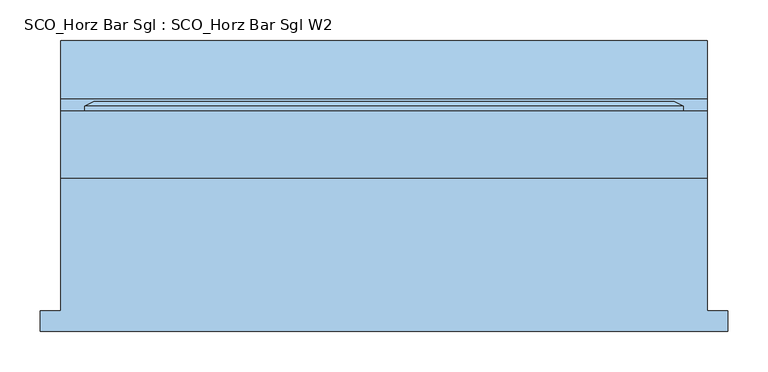
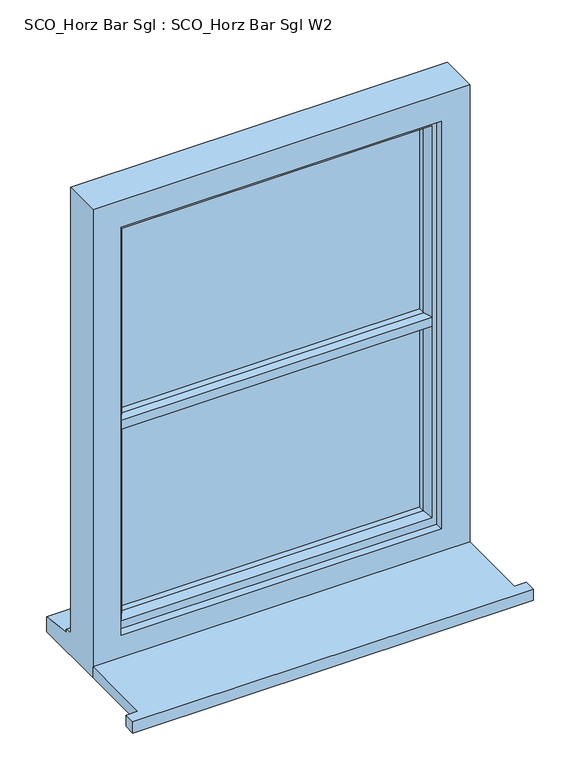
"""IFC4 building model written with IfcOpenShell, lengths in millimetres: window geometry, SCO_Horz Bar Sgl : SCO_Horz Bar Sgl W2."""

from ifc_helpers import new_model, si_unit, frame, origin, place, context, project, spatial, polyline, outline, extrude, faceted_brep, source, transform, mapped, element, save


def sco_horz_bar_sgl_sco_horz_bar_sgl_w2_7f5f4811(model_context):
    return source(origin(), model_context, "Body", "SolidModel", [
        extrude(outline(polyline([(-425.0, -191.5434322), (-425.0, -166.5434322), (-400.0, -166.5434322), (-400.0, -2.0434322), (400.0, -2.0434322), (400.0, -166.5434322), (425.0, -166.5434322), (425.0, -191.5434322), (-425.0, -191.5434322)])), frame((0.0, 0.0, 1060.0), z_axis=(0.0, 0.0, 1.0), x_axis=(1.0, 0.0, 0.0)), (0.0, 0.0, 1.0), 25.0),
        faceted_brep([(-400.0, -2.0434322, 1060.0), (400.0, -2.0434322, 1060.0), (400.0, -2.0434322, 2110.0), (-400.0, -2.0434322, 2110.0), (-340.0, -2.0434322, 2050.0), (340.0, -2.0434322, 2050.0), (340.0, -2.0434322, 1135.0), (-340.0, -2.0434322, 1135.0), (-400.0, 80.9565678, 2110.0), (-400.0, 80.9565678, 1111.0), (-400.0, 95.9565678, 1109.68767), (-400.0, 95.9565678, 1104.7449676), (-400.0, 168.4565678, 1093.8088847), (-400.0, 168.4565678, 1060.0), (400.0, 80.9565678, 2110.0), (400.0, 80.9565678, 1111.0), (-360.0, 80.9565678, 2070.0), (-360.0, 80.9565678, 1123.0), (360.0, 80.9565678, 1123.0), (360.0, 80.9565678, 2070.0), (-360.0, 15.9565678, 2070.0), (-360.0, 15.9565678, 1123.0), (360.0, 15.9565678, 2070.0), (360.0, 15.9565678, 1123.0), (-340.0, 15.9565678, 2050.0), (-340.0, 15.9565678, 1135.0), (340.0, 15.9565678, 1135.0), (340.0, 15.9565678, 2050.0), (400.0, 168.4565678, 1060.0), (400.0, 168.4565678, 1093.8088847), (400.0, 95.9565678, 1104.7449676), (400.0, 95.9565678, 1109.68767)], [[[0, 1, 2, 3], [4, 5, 6, 7]], [[0, 3, 8, 9, 10, 11, 12, 13]], [[9, 8, 14, 15], [16, 17, 18, 19]], [[17, 16, 20, 21]], [[20, 22, 23, 21], [24, 25, 26, 27]], [[24, 4, 7, 25]], [[3, 2, 14, 8]], [[16, 19, 22, 20]], [[5, 4, 24, 27]], [[15, 14, 2, 1, 28, 29, 30, 31]], [[19, 18, 23, 22]], [[5, 27, 26, 6]], [[28, 1, 0, 13]], [[29, 28, 13, 12]], [[30, 29, 12, 11]], [[31, 30, 11, 10]], [[15, 31, 10, 9]], [[21, 23, 18, 17]], [[7, 6, 26, 25]]]),
        extrude(outline(polyline([(330.1480377, 44.9565678), (-330.0, 44.9565678), (-330.0, 68.9565678), (330.1480377, 68.9565678), (330.1480377, 44.9565678)])), frame((0.0, 0.0, 1153.0), z_axis=(0.0, 0.0, 1.0), x_axis=(1.0, 0.0, 0.0)), (0.0, 0.0, 1.0), 434.3307627),
        extrude(outline(polyline([(330.1480377, 44.9565678), (-330.0, 44.9565678), (-330.0, 68.9565678), (330.1480377, 68.9565678), (330.1480377, 44.9565678)])), frame((0.0, 0.0, 1597.6692373), z_axis=(0.0, 0.0, 1.0), x_axis=(1.0, 0.0, 0.0)), (0.0, 0.0, 1.0), 442.3307627),
        extrude(outline(polyline([(92.5035732, 1597.6692373), (92.5035732, 1587.3307627), (86.8277797, 1577.5), (68.9565678, 1577.5), (68.9565678, 1584.5), (44.9565678, 1584.5), (44.9565678, 1577.5), (30.4494677, 1577.5), (15.9565678, 1582.6480377), (15.9565678, 1602.3519623), (30.4494677, 1607.5), (44.9565678, 1607.5), (44.9565678, 1600.5), (68.9565678, 1600.5), (68.9565678, 1607.5), (86.8277797, 1607.5), (92.5035732, 1597.6692373)])), frame((-330.1480377, 0.0, 0.0), z_axis=(1.0, 0.0, 0.0), x_axis=(0.0, 1.0, 0.0)), (0.0, 0.0, 1.0), 660.2960754),
        faceted_brep([(-370.0, 80.9565678, 2072.0), (-370.0, 86.7300705, 2072.0), (-370.0, 86.7300705, 1113.0), (-370.0, 80.9565678, 1113.0), (-360.0, 15.9565678, 2062.0), (-360.0, 80.9565678, 2062.0), (-360.0, 80.9565678, 1123.0), (-360.0, 15.9565678, 1123.0), (-320.0, 30.4494677, 2022.0), (-330.1480377, 15.9565678, 2032.1480377), (-330.1480377, 15.9565678, 1152.8519623), (-320.0, 30.4494677, 1163.0), (-320.0, 44.9565678, 2022.0), (-320.0, 44.9565678, 1163.0), (-330.0, 68.9565678, 2032.0), (-330.0, 44.9565678, 2032.0), (-330.0, 44.9565678, 1153.0), (-330.0, 68.9565678, 1153.0), (-320.0, 86.7300705, 2022.0), (-320.0, 68.9565678, 2022.0), (-320.0, 68.9565678, 1163.0), (-320.0, 86.7300705, 1163.0), (-330.0, 92.5035732, 2032.0), (-330.0, 92.5035732, 1153.0), (-359.2153903, 92.5035732, 2061.2153903), (-359.2153903, 92.5035732, 1123.7846097), (370.0, 86.7300705, 1113.0), (370.0, 80.9565678, 1113.0), (360.0, 80.9565678, 1123.0), (360.0, 15.9565678, 1123.0), (330.1480377, 15.9565678, 1152.8519623), (320.0, 30.4494677, 1163.0), (320.0, 44.9565678, 1163.0), (330.0, 44.9565678, 1153.0), (330.0, 68.9565678, 1153.0), (320.0, 68.9565678, 1163.0), (320.0, 86.7300705, 1163.0), (330.0, 92.5035732, 1153.0), (359.2153903, 92.5035732, 1123.7846097), (370.0, 86.7300705, 2072.0), (370.0, 80.9565678, 2072.0), (360.0, 80.9565678, 2062.0), (360.0, 15.9565678, 2062.0), (330.1480377, 15.9565678, 2032.1480377), (320.0, 30.4494677, 2022.0), (320.0, 44.9565678, 2022.0), (330.0, 44.9565678, 2032.0), (330.0, 68.9565678, 2032.0), (320.0, 68.9565678, 2022.0), (320.0, 86.7300705, 2022.0), (330.0, 92.5035732, 2032.0), (359.2153903, 92.5035732, 2061.2153903)], [[[0, 1, 2, 3]], [[4, 5, 6, 7]], [[8, 9, 10, 11]], [[12, 8, 11, 13]], [[14, 15, 16, 17]], [[18, 19, 20, 21]], [[22, 18, 21, 23]], [[1, 24, 25, 2]], [[3, 2, 26, 27]], [[7, 6, 28, 29]], [[11, 10, 30, 31]], [[13, 11, 31, 32]], [[17, 16, 33, 34]], [[21, 20, 35, 36]], [[23, 21, 36, 37]], [[2, 25, 38, 26]], [[27, 26, 39, 40]], [[29, 28, 41, 42]], [[31, 30, 43, 44]], [[32, 31, 44, 45]], [[34, 33, 46, 47]], [[36, 35, 48, 49]], [[37, 36, 49, 50]], [[26, 38, 51, 39]], [[40, 39, 1, 0]], [[3, 27, 40, 0], [5, 41, 28, 6]], [[42, 41, 5, 4]], [[7, 29, 42, 4], [9, 43, 30, 10]], [[44, 43, 9, 8]], [[45, 44, 8, 12]], [[15, 46, 33, 16], [13, 32, 45, 12]], [[47, 46, 15, 14]], [[17, 34, 47, 14], [19, 48, 35, 20]], [[49, 48, 19, 18]], [[50, 49, 18, 22]], [[24, 51, 38, 25], [23, 37, 50, 22]], [[39, 51, 24, 1]]]),
    ])


if __name__ == "__main__":
    model = new_model("IFC4")
    model_context = context("Model", 3, world=origin())
    ifc_project = project(units=[si_unit("LENGTHUNIT", "METRE", prefix="MILLI")], contexts=[model_context])
    site = spatial("IfcSite", under=ifc_project)
    building = spatial("IfcBuilding", under=site)
    placement = place(None, origin())
    sco_horz_bar_sgl_sco_horz_bar_sgl_w2_shape = sco_horz_bar_sgl_sco_horz_bar_sgl_w2_7f5f4811(model_context)
    element("IfcWindow", 1, ObjectType="SCO_Horz Bar Sgl : SCO_Horz Bar Sgl W2", at=placement, inside=building, context=model_context, shape_type="MappedRepresentation", body=[
        mapped(sco_horz_bar_sgl_sco_horz_bar_sgl_w2_shape, transform((0.0, 0.0, 0.0), x_axis=(1.0, 0.0, 0.0), y_axis=(0.0, 1.0, 0.0), z_axis=(0.0, 0.0, 1.0))),
    ])
    save(model, "model.ifc")

# Revit data of these elements
# Type "SCO_Horz Bar Sgl : SCO_Horz Bar Sgl W2"
#   Type Mark = "W2"
#   Operation = "SinglePanel"
#   Manufacturer = "Revit"
#   Keynote = "L10"
#   Wrap Layers (Ext) from Ext = 102.5 mm
#   Wrap Layers (Int) from Ext = 177.5 mm
#   Window Board Projection = 25 mm
#   Window Board Extension = 25 mm
#   Rough Width = 800 mm
#   Rough Height = 1050 mm
#   Height = 1050 mm
#   Width = 800 mm
#   Glazing Thickness = 24 mm
#   FrameOffset - External = 102.5 mm
#   Frame Depth = 65 mm
#   Ext Leaf Thickness (Scot) = 102.5 mm
#   Ext Leaf Overlap (Scot) = 25 mm
#   Default Head Height = 2110 mm
#   Cill Depth = 87.5 mm
#   Cavity Closer Width = 50 mm
#   Cavity Closer Offset from Ext = 102.5 mm
#   Cavity Closer Depth = 85 mm
#   Vis - Cavity Closers = yes
#   Material Trim = Window Frame
#   Material Glass = Glass
#   Material Frame = Window Frame
#   Wall Closure = (empty or 0)
# Element 1 (IfcWindow, "SCO_Horz Bar Sgl : SCO_Horz Bar Sgl W2")
#   Materials on its faces: "Window Frame", "Glass"
# Materials
#   "Window Frame": class "Miscellaneous", colour RGB 249 249 249, transparency 0
#   "Glass": class "Glass", colour RGB 0 128 192, transparency 0.75
